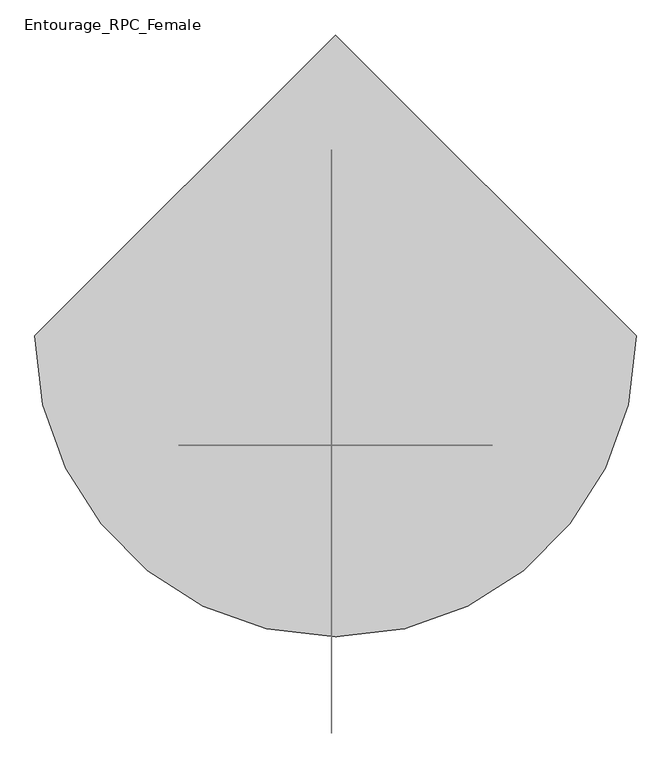
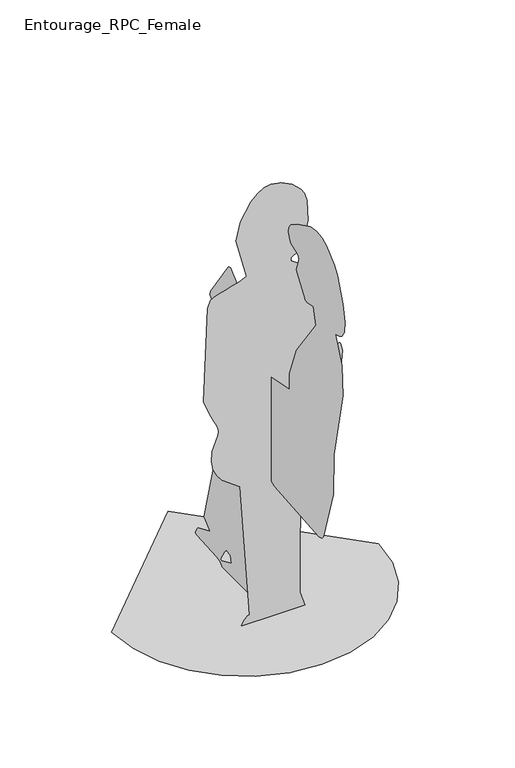
"""IFC4 building model written with IfcOpenShell, lengths in millimetres: proxy geometry, Entourage_RPC_Female : Cynthia."""

from ifc_helpers import new_model, si_unit, origin, place, context, project, spatial, triangles, source, transform, mapped, element, save


def entourage_rpc_female_c3b5a3e1(model_context):
    return source(origin(), model_context, "Body", "Tessellation", [
        triangles([(-437.3060472, 0.0, 2.93e-05), (-425.7451249, -100.2016327, 2.93e-05), (-392.8196637, -192.220807, 2.93e-05), (-341.1660942, -273.421065, 2.93e-05), (-273.4210832, -341.1661669, 2.93e-05), (-192.2207525, -392.8196274, 2.93e-05), (-100.2015873, -425.7450522, 2.93e-05), (1.91e-05, -437.3060472, 2.93e-05), (100.2016418, -425.7451249, 2.93e-05), (192.2208252, -392.8196637, 2.93e-05), (273.4210832, -341.1660942, 2.93e-05), (341.1662395, -273.4210832, 2.93e-05), (392.8196274, -192.2207344, 2.93e-05), (425.7450522, -100.2015691, 2.93e-05), (437.3060472, 3.36e-05, 2.93e-05), (-5.73e-05, 437.3060835, 2.93e-05), (-5.5814595, 72.2469164, 69.4963894), (-5.5814595, 67.0311828, 46.0256926), (-5.5814618, 124.4040072, 19.9471473), (-5.5814618, 129.6197135, 25.1628355), (-5.5814606, 107.6002908, 62.2269748), (-5.5814595, 95.7176132, 74.7120821), (-5.5814595, -28.6037251, 4.4e-06), (-5.5814589, -39.8908927, 35.5942709), (-5.5814589, -42.4985824, 37.2668455), (-5.5814583, -45.6386024, 39.1828236), (-5.5814583, -48.9915681, 41.1595925), (-5.5814583, -52.2381586, 43.0148617), (-5.5814583, -55.0589485, 44.5657618), (-5.5814583, -57.1346439, 45.630268), (-5.5814583, -58.1458422, 46.0256972), (-5.5814595, -58.1459239, 5.3e-06), (-5.5814589, -108.9534877, 6.8e-06), (-5.5814578, -116.5758876, 29.8220396), (-5.5814544, -109.3237594, 163.617066), (-5.5814447, -45.4571863, 488.7460396), (-5.5814447, -47.7144613, 510.22398), (-5.5814447, -52.930154, 512.8317787), (-5.5814442, -176.693648, 461.1355883), (-5.5814407, -431.0103195, 441.4519423), (-5.5814407, -446.7163739, 445.0275962), (-5.5814402, -456.1588572, 455.8254473), (-5.5814334, -511.6812675, 636.0533998), (-5.5814294, -514.5206291, 776.2252218), (-5.581422, -566.7675127, 1012.4535353), (-5.5814192, -561.4620226, 1112.6385538), (-5.5814163, -522.3441341, 1198.6978357), (-5.5814163, -544.766203, 1204.597403), (-5.5814158, -561.2101121, 1214.9823069), (-5.5814152, -573.9146782, 1236.2579704), (-5.5814135, -577.4590839, 1272.8749214), (-5.5814124, -566.4222939, 1329.2833969), (-5.5814107, -535.3834182, 1409.9341427), (-5.5814101, -516.7875329, 1433.7646648), (-5.5814095, -472.5757693, 1474.3213463), (-5.5814095, -445.9834971, 1486.7823589), (-5.5814101, -415.7492961, 1491.1889214), (-5.5814107, -381.3848602, 1485.4078789), (-5.5814124, -308.1104447, 1450.1712215), (-5.5814135, -271.6909563, 1426.3745636), (-5.5814141, -259.9824413, 1410.5522736), (-5.5814152, -256.5010404, 1391.3537361), (-5.5814158, -264.1664701, 1368.2083466), (-5.5814158, -270.5527808, 1361.5173306), (-5.5814158, -307.4895524, 1345.9739479), (-5.5814158, -313.689719, 1341.0972107), (-5.5814158, -316.3235335, 1334.3062008), (-5.5814163, -314.5106718, 1321.5905525), (-5.5814175, -303.2843222, 1289.972715), (-5.5814175, -303.9330653, 1281.3193188), (-5.5814186, -344.8554039, 1227.4574902), (-5.5814192, -350.225752, 1216.9527534), (-5.5814192, -354.0102593, 1213.1380154), (-5.5814192, -360.9106739, 1211.8318451), (-5.581418, -397.1671454, 1216.9527534), (-5.5814197, -412.8142282, 1162.1877823), (-5.5814254, -300.7219422, 1007.465613), (-5.5814294, -262.9223781, 903.7025425), (-5.5814311, -261.5586532, 849.245256), (-5.5814334, -151.2455011, 828.1027239), (-5.5814334, -131.1658673, 828.382358), (-5.5814322, -146.9134072, 873.4852736), (-5.5814322, -146.8129955, 875.3236788), (-5.5814322, -136.528476, 880.5995195), (-5.5814294, 66.2908937, 1062.7625284), (-5.5814294, 72.9542315, 1068.1179428), (-5.58143, 85.3176393, 1063.7725685), (-5.5814356, 186.9121194, 916.7362673), (-5.5814362, 189.6004001, 904.0100819), (-5.5814373, 74.8547605, 802.3037899), (-5.5814385, 53.5232047, 768.5295433), (-5.5814385, 40.9526375, 757.9702314), (-5.5814385, 7.0502453, 750.1467264), (-5.5814396, -30.7395867, 681.3431499), (-5.5814396, -32.0672991, 677.1266922), (-5.5814402, -2.7970188, 673.1422697), (-5.5814413, 74.8547605, 666.6952068), (-5.5814606, 223.5024732, 113.8299342), (-5.5814606, 192.3028696, 86.4272827), (-5.5814606, 189.6004001, 82.5356507), (-5.5814629, 257.4046916, 53.8492703), (-5.5814629, 261.0574302, 50.6335736), (-5.5814635, 266.9933869, 41.9573681), (-5.5814635, 270.402463, 33.1798516), (-5.5814635, 270.8967278, 29.8373366), (-5.5814635, 270.4438667, 27.7706795), (-5.5814635, 262.2121017, 24.672413), (-5.5814623, 148.399036, 17.7234889), (-5.5814623, 129.6197135, 12.1235673), (-5.5814623, 119.228015, 0.0), (-103.2161744, -158.8626324, 3.1383159), (-93.5649829, -158.8626324, 19.2429933), (-88.6212531, -158.8626324, 24.4594445), (-82.9718341, -158.8626324, 28.4095327), (-76.7114059, -158.8626324, 30.3785123), (-108.0056803, -158.8626688, 484.1452303), (-166.5179246, -158.8626688, 527.9972775), (-183.6323596, -158.8626688, 549.7335234), (-196.1560501, -158.8626688, 575.2326937), (-202.051348, -158.8626688, 604.6170193), (-199.2806414, -158.8626688, 638.0087311), (-180.7338447, -158.8626688, 688.9253906), (-179.5105545, -158.8626688, 700.1741953), (-181.0256691, -158.8626688, 711.0286926), (-186.0299967, -158.8626688, 724.8032879), (-192.7432497, -158.8626688, 739.7140783), (-208.556347, -158.8626688, 771.7153954), (-227.9670263, -158.8626688, 820.5585623), (-215.5927998, -158.8627051, 1139.719677), (-204.4963295, -158.8627051, 1164.795472), (-195.7042972, -158.8627051, 1170.2251551), (-178.3999392, -158.8627051, 1176.5906822), (-156.0961225, -158.8627051, 1183.4371393), (-132.3056233, -158.8627051, 1190.3085222), (-110.5413813, -158.8627051, 1196.7500622), (-94.3161544, -158.8627051, 1202.3061911), (-87.1428368, -158.8627051, 1206.5211954), (-121.0449553, -158.8627051, 1339.5217255), (-105.9598841, -158.8627233, 1402.4776211), (-72.2006802, -158.8627233, 1459.3937691), (-51.1399244, -158.8627233, 1480.6096252), (-28.7965753, -158.8627233, 1494.3423626), (-6.2993163, -158.8627233, 1498.6009689), (28.3786116, -158.8627233, 1491.3014145), (62.9444138, -158.8627233, 1473.3404469), (92.2084978, -158.8627233, 1445.5319698), (103.2306357, -158.8627233, 1428.1888424), (112.1217082, -158.8627233, 1400.9906479), (114.2135863, -158.8627051, 1329.2272957), (96.1615087, -158.8627051, 1258.9099308), (79.8726138, -158.8627051, 1233.5191841), (58.8970909, -158.8627051, 1219.5604431), (58.8970909, -158.8627051, 1209.1289577), (105.4403209, -158.8627051, 1177.1577988), (186.6819918, -158.8627051, 1146.5404089), (190.9102947, -158.8627051, 1130.2535397), (197.4606216, -158.8627051, 874.561952), (217.1153449, -158.8627051, 870.6129925), (219.4355885, -158.8627051, 869.5271576), (221.3550207, -158.8627051, 866.9867603), (227.9670444, -158.8626688, 839.7671282), (217.976248, -158.8626688, 726.675848), (216.7788284, -158.8626688, 725.5374001), (198.4189752, -158.8626688, 721.3537165), (197.1134226, -158.8626688, 721.4601053), (188.2935758, -158.8626688, 736.0854481), (176.2505791, -158.8626688, 750.1465811), (172.5435924, -158.8626688, 744.3788372), (169.4577161, -158.8626688, 737.624235), (166.7655839, -158.8626688, 730.2871828), (164.2398296, -158.8626688, 722.7722345), (161.6531779, -158.8626688, 715.4839439), (158.7782626, -158.8626688, 708.8267195), (155.3877173, -158.8626688, 703.2051149), (164.598892, -158.8626688, 582.3868355), (159.7289131, -158.8626688, 557.9940293), (150.1720292, -158.8626688, 536.3024028), (143.4522449, -158.8626688, 528.6089407), (105.4337806, -158.8626688, 509.5450607), (96.8766176, -158.8626688, 503.2558007), (90.1913244, -158.8626688, 494.5766793), (88.7456459, -158.8626324, 49.410397), (105.4366693, -158.8626324, 7.4e-05), (-104.3910663, -158.8626324, 7.4e-05)], [[15, 16, 1], [14, 15, 1], [14, 1, 2], [13, 14, 2], [13, 2, 3], [13, 3, 4], [12, 13, 4], [11, 12, 4], [11, 4, 5], [11, 5, 6], [11, 6, 7], [11, 7, 8], [11, 8, 9], [11, 9, 10], [23, 17, 18], [110, 23, 18], [110, 18, 19], [109, 110, 19], [17, 23, 24], [31, 32, 33], [31, 33, 34], [109, 19, 20], [108, 109, 20], [88, 89, 90], [82, 83, 84], [85, 86, 87], [105, 106, 107], [104, 105, 107], [103, 104, 107], [102, 103, 107], [101, 102, 107], [100, 101, 107], [100, 107, 108], [100, 108, 20], [100, 20, 21], [100, 21, 22], [87, 88, 90], [85, 87, 90], [84, 85, 90], [84, 90, 91], [84, 91, 92], [84, 92, 93], [82, 84, 93], [81, 82, 93], [81, 93, 94], [80, 81, 94], [80, 94, 95], [99, 100, 22], [17, 24, 25], [17, 25, 26], [31, 34, 35], [30, 31, 35], [17, 26, 27], [17, 27, 28], [17, 28, 29], [29, 30, 35], [17, 29, 35], [22, 17, 35], [99, 22, 35], [98, 99, 35], [97, 98, 35], [97, 35, 36], [97, 36, 37], [96, 97, 37], [96, 37, 38], [95, 96, 38], [80, 95, 38], [80, 38, 39], [79, 80, 39], [79, 39, 40], [79, 40, 41], [79, 41, 42], [79, 42, 43], [79, 43, 44], [78, 79, 44], [77, 78, 44], [77, 44, 45], [77, 45, 46], [76, 77, 46], [76, 46, 47], [75, 76, 47], [72, 73, 74], [71, 72, 74], [61, 62, 63], [60, 61, 63], [60, 63, 64], [59, 60, 64], [59, 64, 65], [59, 65, 66], [58, 59, 66], [57, 58, 66], [56, 57, 66], [55, 56, 66], [54, 55, 66], [54, 66, 67], [53, 54, 67], [52, 53, 67], [52, 67, 68], [51, 52, 68], [50, 51, 68], [49, 50, 68], [48, 49, 68], [47, 48, 68], [75, 47, 68], [74, 75, 68], [71, 74, 68], [70, 71, 68], [69, 70, 68], [183, 184, 111], [183, 111, 112], [183, 112, 113], [183, 113, 114], [183, 114, 115], [182, 183, 115], [181, 182, 115], [181, 115, 116], [154, 155, 156], [164, 165, 166], [180, 181, 116], [163, 164, 166], [162, 163, 166], [162, 166, 167], [161, 162, 167], [160, 161, 167], [159, 160, 167], [158, 159, 167], [157, 158, 167], [180, 116, 117], [180, 117, 118], [180, 118, 119], [180, 119, 120], [180, 120, 121], [180, 121, 122], [179, 180, 122], [179, 122, 123], [178, 179, 123], [177, 178, 123], [176, 177, 123], [175, 176, 123], [174, 175, 123], [174, 123, 124], [174, 124, 125], [173, 174, 125], [172, 173, 125], [171, 172, 125], [170, 171, 125], [169, 170, 125], [169, 125, 126], [168, 169, 126], [168, 126, 127], [167, 168, 127], [157, 167, 127], [157, 127, 128], [156, 157, 128], [154, 156, 128], [153, 154, 128], [153, 128, 129], [153, 129, 130], [153, 130, 131], [153, 131, 132], [153, 132, 133], [153, 133, 134], [153, 134, 135], [153, 135, 136], [153, 136, 137], [152, 153, 137], [151, 152, 137], [150, 151, 137], [149, 150, 137], [149, 137, 138], [149, 138, 139], [148, 149, 139], [147, 148, 139], [146, 147, 139], [146, 139, 140], [145, 146, 140], [145, 140, 141], [144, 145, 141], [144, 141, 142], [144, 142, 143]], closed=False),
    ])


if __name__ == "__main__":
    model = new_model("IFC4")
    model_context = context("Model", 3, world=origin())
    ifc_project = project(units=[si_unit("LENGTHUNIT", "METRE", prefix="MILLI")], contexts=[model_context])
    site = spatial("IfcSite", under=ifc_project)
    building = spatial("IfcBuilding", under=site)
    placement = place(None, origin())
    entourage_rpc_female_shape = entourage_rpc_female_c3b5a3e1(model_context)
    element("IfcBuildingElementProxy", 1, Name="Entourage_RPC_Female : Cynthia", ObjectType="Entourage_RPC_Female : Cynthia", at=placement, inside=building, context=model_context, shape_type="MappedRepresentation", body=[
        mapped(entourage_rpc_female_shape, transform((0.0, 0.0, 0.0), x_axis=(1.0, 0.0, 0.0), y_axis=(0.0, 1.0, 0.0), z_axis=(0.0, 0.0, 1.0))),
    ])
    save(model, "model.ifc")

# Revit data of these elements
# Type "Entourage_RPC_Female : Cynthia"
#   built-in parameter 1005198 = "{2, 15},{22, RPC-8-FXA2-QQQ0-UGV2-6},{1, 0},{1, 0},{2, 15},{1, 8},{5, Color},{1, 0},{1, 0},{3, 0.8},{3, 0.8},{3, 0.8},{1, 8},{7, BBoxMin},{1, 0},{1, 0},{1, 0},{1, 0},{1, 0},{1, 8},{7, BBoxMax},{1, 0},{1, 0},{1, 0},{1, 0},{1, 0},{2, 11},{9, RPCTypeId},{1, 0},{1, 0},{22, RPC-8-FXA2-QQQ0-UGV2-6},{1, 6},{14, RPCPlantHeight},{1, 0},{1, 0},{7, 4.91667},{2, 11},{7, keyword},{1, 0},{1, 0},{43, :RPCs:People [Seated-Business]:Geometry:RPC},{2, 11},{8, category},{1, 0},{1, 0},{24, People [Seated-Business]},{2, 11},{12, LocalizedUID},{1, 0},{1, 0},{7, Cynthia},{2, 14},{6, Height},{1, 0},{1, 0},{7, 4.91667},{1, 2},{16, Cast Reflections},{1, 0},{1, 0},{1, 0},{1, 2},{6, Jitter},{1, 0},{1, 0},{1, 1},{1, 2},{9, Billboard},{1, 0},{1, 0},{1, 0},{1, 2},{12, Cast Shadows},{1, 0},{1, 0},{1, 1},{1, 2},{20, Apply Filter Effects},{1, 0},{1, 0},{1, 0},{2, 11},{28, Apply Filter Effects-Text-FC},{1, 0},{1, 0},{4, None},{21, assetlibrary_base.fbx},{1, 5},"
#   built-in parameter 1005195 = "RPC-8-FXA2-QQQ0-UGV2-6"
#   Height = 0
